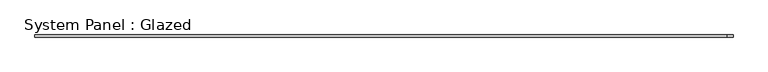
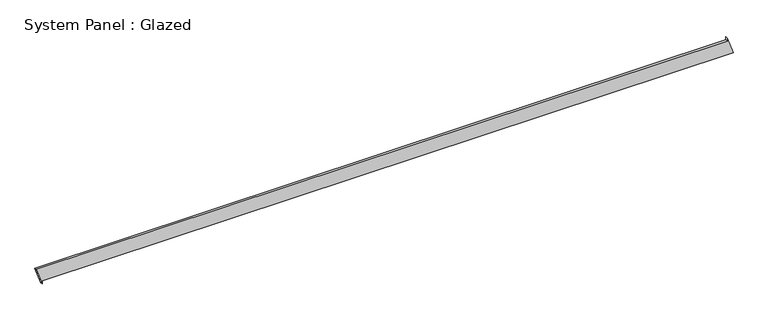
"""IFC4 building model written with IfcOpenShell, lengths in millimetres: plate geometry, System Panel : Glazed."""

from ifc_helpers import new_model, si_unit, frame, origin, place, context, project, spatial, polyline, outline, extrude, source, transform, mapped, element, save


def system_panel_glazed_13b512fd(model_context):
    return source(origin(), model_context, "Body", "SweptSolid", [
        extrude(outline(polyline([(0.0, -3959.20642), (35.3553391, -3959.20642), (35.3553391, 4028.228324), (235.5969396, 3959.1733726), (200.2416005, 3959.173312), (200.2552692, -4028.228324), (0.0, -3959.20642)])), frame((0.0, -49.5, 0.0), z_axis=(0.0, 1.0, 0.0), x_axis=(0.0, 0.0, 1.0)), (0.0, 0.0, 1.0), 25.0),
    ])


if __name__ == "__main__":
    model = new_model("IFC4")
    model_context = context("Model", 3, world=origin())
    ifc_project = project(units=[si_unit("LENGTHUNIT", "METRE", prefix="MILLI")], contexts=[model_context])
    site = spatial("IfcSite", under=ifc_project)
    building = spatial("IfcBuilding", under=site)
    placement = place(None, origin())
    system_panel_glazed_shape = system_panel_glazed_13b512fd(model_context)
    element("IfcPlate", 1, ObjectType="System Panel : Glazed", at=placement, inside=building, context=model_context, shape_type="MappedRepresentation", body=[
        mapped(system_panel_glazed_shape, transform((0.0, 0.0, 0.0), x_axis=(1.0, 0.0, 0.0), y_axis=(0.0, 1.0, 0.0), z_axis=(0.0, 0.0, 1.0))),
    ])
    save(model, "model.ifc")

# Revit data of these elements
# Element 1 (IfcPlate, "System Panel : Glazed")
#   Materials on its faces: "Glass"
# Materials
#   "Glass": class "Glass", colour RGB 218 227 224, transparency 0.85, Description = "Soda Lime Glass", Cost = 0
